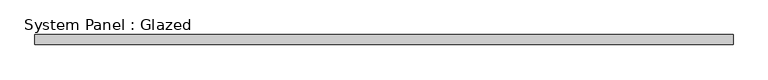
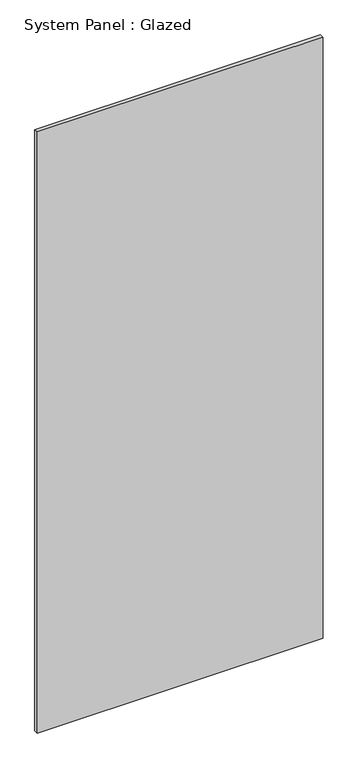
"""IFC4 building model written with IfcOpenShell, lengths in millimetres: plate geometry, System Panel : Glazed."""

from ifc_helpers import new_model, si_unit, origin, origin_with_axes, place, context, project, spatial, polyline, outline, extrude, source, transform, mapped, element, save


def system_panel_glazed_29efa263(model_context):
    return source(origin(), model_context, "Body", "SweptSolid", [
        extrude(outline(polyline([(877.5000002, 24.5), (-877.5000002, 24.5), (-877.5000002, 49.5), (877.5000002, 49.5), (877.5000002, 24.5)])), origin_with_axes(), (0.0, 0.0, 1.0), 3900.0),
    ])


if __name__ == "__main__":
    model = new_model("IFC4")
    model_context = context("Model", 3, world=origin())
    ifc_project = project(units=[si_unit("LENGTHUNIT", "METRE", prefix="MILLI")], contexts=[model_context])
    site = spatial("IfcSite", under=ifc_project)
    building = spatial("IfcBuilding", under=site)
    placement = place(None, origin())
    system_panel_glazed_shape = system_panel_glazed_29efa263(model_context)
    element("IfcPlate", 1, ObjectType="System Panel : Glazed", at=placement, inside=building, context=model_context, shape_type="MappedRepresentation", body=[
        mapped(system_panel_glazed_shape, transform((0.0, 0.0, 0.0), x_axis=(1.0, 0.0, 0.0), y_axis=(0.0, 1.0, 0.0), z_axis=(0.0, 0.0, 1.0))),
    ])
    save(model, "model.ifc")

# Revit data of these elements
# Type "System Panel : Glazed"
#   Keynote = "H11"
#   Construction Type Id = "GSP4R"
#   Analytic Construction = "1/8 in Pilkington single glazing"
#   Visual Light Transmittance = 0.9
#   Solar Heat Gain Coefficient = 0.86
#   Heat Transfer Coefficient (U) = 6.7069 W/(m²·K)
#   Define Thermal Properties by = 1
# Element 1 (IfcPlate, "System Panel : Glazed")
#   Materials on its faces: "Glass"
# Materials
#   "Glass": class "Glass", colour RGB 0 128 192, transparency 0.9, Description = "Soda Lime Glass", Cost = 0
